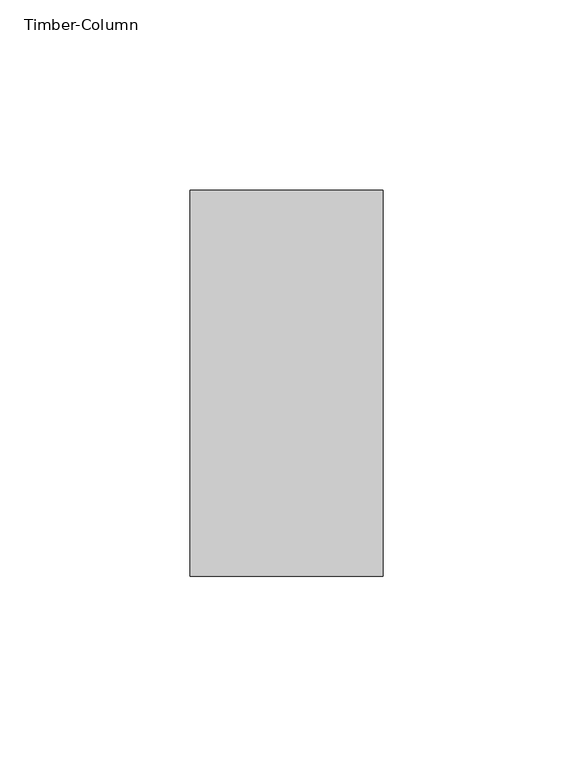
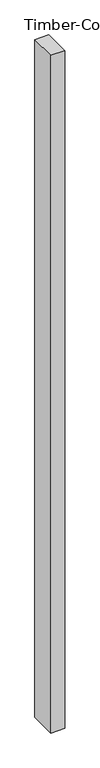
"""IFC4 building model written with IfcOpenShell, lengths in millimetres: column geometry, Timber-Column."""

import ifcopenshell
import ifcopenshell.guid

model = None  # the IFC model being written
_history = None  # IfcOwnerHistory: only IFC2X3 demands one
_inside = {}  # id of a spatial element -> (the spatial element, [elements in it])
_under = {}  # id of a project, library or spatial element -> (it, [spatial elements below it])
_declared = {}  # id of a project -> (the project, [libraries it declares])
_typed = {}  # id of a type object -> (the type object, [elements of that type])
_made_of = {}  # id of a material, layer set ... -> (it, [elements and type objects made of it])


def new_model(schema):
    """Start an empty IFC model of exactly this schema.

    Asked for "IFC4X3", IfcOpenShell would pick the latest addendum, in which some entities
    have other attributes; the version numbers below select the first issue.
    IFC2X3 requires an IfcOwnerHistory on every rooted entity: one is made here for all.
    """
    global model, _history
    if schema == "IFC4X3":
        model = ifcopenshell.file(schema_version=(4, 3, 0, 0))
    else:
        model = ifcopenshell.file(schema=schema)
    _inside.clear()
    _under.clear()
    _declared.clear()
    _typed.clear()
    _made_of.clear()
    _history = None
    if model.schema == "IFC2X3":
        org = make("IfcOrganization", Name="unknown")
        user = make(
            "IfcPersonAndOrganization",
            ThePerson=make("IfcPerson", FamilyName="unknown"),
            TheOrganization=org,
        )
        app = make(
            "IfcApplication",
            ApplicationDeveloper=org,
            Version="unknown",
            ApplicationFullName="unknown",
            ApplicationIdentifier="unknown",
        )
        _history = make(
            "IfcOwnerHistory",
            OwningUser=user,
            OwningApplication=app,
            ChangeAction="ADDED",
            CreationDate=0,
        )
    return model


def make(cls, **values):
    """One entity of the class cls with the attributes given. An attribute that is None is left unset."""
    return model.create_entity(
        cls, **{name: value for name, value in values.items() if value is not None}
    )


def rooted(cls, **values):
    """An entity with a GlobalId (a new one), such as an element, a storey or a relation."""
    return make(cls, GlobalId=ifcopenshell.guid.new(), OwnerHistory=_history, **values)


def si_unit(unit_type, name, prefix=None):
    """IfcSIUnit, for example si_unit("LENGTHUNIT", "METRE", prefix="MILLI")."""
    return make("IfcSIUnit", UnitType=unit_type, Prefix=prefix, Name=name)


def assignment(units):
    """IfcUnitAssignment: the units of a project."""
    return None if units is None else make("IfcUnitAssignment", Units=units)


def point(xyz):
    """IfcCartesianPoint."""
    return None if xyz is None else make("IfcCartesianPoint", Coordinates=xyz)


def direction(xyz):
    """IfcDirection."""
    return None if xyz is None else make("IfcDirection", DirectionRatios=xyz)


def frame(location, z_axis=None, x_axis=None):
    """IfcAxis2Placement3D, a coordinate frame: its origin and axes. An axis left out is left unset."""
    return make(
        "IfcAxis2Placement3D",
        Location=point(location),
        Axis=direction(z_axis),
        RefDirection=direction(x_axis),
    )


def origin():
    """The frame at (0, 0, 0) with its axes left unset."""
    return frame((0.0, 0.0, 0.0))


def place(relative_to, where):
    """IfcLocalPlacement: puts the frame where relative to a parent placement (None: the world)."""
    return make(
        "IfcLocalPlacement", PlacementRelTo=relative_to, RelativePlacement=where
    )


def context(
    kind, dimensions, precision=None, world=None, true_north=None, identifier=None
):
    """IfcGeometricRepresentationContext, for example the 3D "Model" context."""
    return make(
        "IfcGeometricRepresentationContext",
        ContextIdentifier=identifier,
        ContextType=kind,
        CoordinateSpaceDimension=dimensions,
        Precision=precision,
        WorldCoordinateSystem=world,
        TrueNorth=true_north,
    )


def project(units=None, contexts=None):
    """IfcProject with its units and contexts."""
    return rooted(
        "IfcProject",
        Name="project",
        RepresentationContexts=contexts,
        UnitsInContext=assignment(units),
    )


def spatial(cls, under=None, at=None, **own):
    """A site, building, storey or space (cls), placed at a placement, below another one or the project."""
    s = rooted(cls, ObjectPlacement=at, **own)
    if under is not None:
        _under.setdefault(under.id(), (under, []))[1].append(s)
    return s


def polyline(points):
    """IfcPolyline through the points."""
    return make("IfcPolyline", Points=[point(p) for p in points])


def outline(outer, holes=None, kind="AREA"):
    """IfcArbitraryClosedProfileDef: a profile drawn as a closed curve; with holes, ...WithVoids."""
    if holes is None:
        return make("IfcArbitraryClosedProfileDef", ProfileType=kind, OuterCurve=outer)
    return make(
        "IfcArbitraryProfileDefWithVoids",
        ProfileType=kind,
        OuterCurve=outer,
        InnerCurves=holes,
    )


def extrude(swept, where, along, depth):
    """IfcExtrudedAreaSolid: the profile swept, set in the frame where, extruded along a direction by depth."""
    return make(
        "IfcExtrudedAreaSolid",
        SweptArea=swept,
        Position=where,
        ExtrudedDirection=direction(along),
        Depth=depth,
    )


def shape(context_of_items, identifier, shape_type, items):
    """IfcShapeRepresentation: the items that make up one representation, for example the "Body"."""
    return make(
        "IfcShapeRepresentation",
        ContextOfItems=context_of_items,
        RepresentationIdentifier=identifier,
        RepresentationType=shape_type,
        Items=items,
    )


def source(mapping_origin, context_of_items, identifier, shape_type, items):
    """IfcRepresentationMap: a shape defined once, which mapped items show again and again."""
    return make(
        "IfcRepresentationMap",
        MappingOrigin=mapping_origin,
        MappedRepresentation=shape(context_of_items, identifier, shape_type, items),
    )


def transform(
    local_origin,
    x_axis=None,
    y_axis=None,
    z_axis=None,
    scale=None,
    scale2=None,
    scale3=None,
    uniform=True,
):
    """IfcCartesianTransformationOperator3D, or its non-uniform kind. x_axis, y_axis, z_axis: its Axis1, 2, 3."""
    if uniform:
        return make(
            "IfcCartesianTransformationOperator3D",
            Axis1=direction(x_axis),
            Axis2=direction(y_axis),
            LocalOrigin=point(local_origin),
            Scale=scale,
            Axis3=direction(z_axis),
        )
    return make(
        "IfcCartesianTransformationOperator3DnonUniform",
        Axis1=direction(x_axis),
        Axis2=direction(y_axis),
        LocalOrigin=point(local_origin),
        Scale=scale,
        Axis3=direction(z_axis),
        Scale2=scale2,
        Scale3=scale3,
    )


def mapped(mapping_source, mapping_target):
    """IfcMappedItem: shows the shape of a source again, moved by a transform."""
    return make(
        "IfcMappedItem", MappingSource=mapping_source, MappingTarget=mapping_target
    )


def made_of(thing, what):
    """Note that an element or type object is made of a material, layer set ...; save() writes the relation."""
    if what is not None:
        _made_of.setdefault(what.id(), (what, []))[1].append(thing)
    return thing


def element(
    cls,
    number,
    at=None,
    inside=None,
    cuts=None,
    type_object=None,
    material=None,
    context=None,
    identifier="Body",
    shape_type=None,
    held_by="IfcProductDefinitionShape",
    body=None,
    shapes=None,
    **own,
):
    """One element of the class cls, such as IfcWall. Its Tag is "e" and its number.

    at: its placement. inside: the storey or other place that contains it. cuts: it is an
    opening in that element (IfcRelVoidsElement). A single representation is given by context,
    identifier, shape_type and body (its items); several are given by shapes. held_by: the class
    of the entity that holds the representations. save() writes the other relations.
    """
    e = rooted(cls, Tag="e%d" % number, ObjectPlacement=at, **own)
    if body is not None:
        shapes = [shape(context, identifier, shape_type, body)]
    if shapes is not None:
        e.Representation = make(held_by, Representations=shapes)
    if inside is not None:
        _inside.setdefault(inside.id(), (inside, []))[1].append(e)
    if cuts is not None:
        rooted(
            "IfcRelVoidsElement", RelatingBuildingElement=cuts, RelatedOpeningElement=e
        )
    if type_object is not None:
        _typed.setdefault(type_object.id(), (type_object, []))[1].append(e)
    return made_of(e, material)


def aggregate(whole, parts):
    """IfcRelAggregates: a whole, such as a stair, and the parts it consists of."""
    return rooted("IfcRelAggregates", RelatingObject=whole, RelatedObjects=parts)


def save(model, path):
    """Write the relations noted so far, then the file.

    IfcRelAggregates (storeys below a building ...), IfcRelContainedInSpatialStructure (elements
    in a storey), IfcRelDefinesByType, IfcRelAssociatesMaterial and IfcRelDeclares: one each for
    every whole, place, type object, material and project.
    """
    for whole, parts in _under.values():
        aggregate(whole, parts)
    for where, things in _inside.values():
        rooted(
            "IfcRelContainedInSpatialStructure",
            RelatedElements=things,
            RelatingStructure=where,
        )
    for kind, things in _typed.values():
        rooted("IfcRelDefinesByType", RelatedObjects=things, RelatingType=kind)
    for what, things in _made_of.values():
        rooted("IfcRelAssociatesMaterial", RelatedObjects=things, RelatingMaterial=what)
    for by, libraries in _declared.values():
        rooted("IfcRelDeclares", RelatingContext=by, RelatedDefinitions=libraries)
    model.write(path)


def timber_column_c014de30(model_context):
    return source(origin(), model_context, "Body", "SweptSolid", [
        extrude(outline(polyline([(25.4, -50.8), (-25.4, -50.8), (-25.4, 50.8), (25.4, 50.8), (25.4, -50.8)])), frame((0.0, 0.0, 50.8), z_axis=(0.0, 0.0, 1.0), x_axis=(1.0, 0.0, 0.0)), (0.0, 0.0, 1.0), 2616.2),
    ])


if __name__ == "__main__":
    model = new_model("IFC4")
    model_context = context("Model", 3, world=origin())
    ifc_project = project(units=[si_unit("LENGTHUNIT", "METRE", prefix="MILLI")], contexts=[model_context])
    site = spatial("IfcSite", under=ifc_project)
    building = spatial("IfcBuilding", under=site)
    placement = place(None, origin())
    timber_column_shape = timber_column_c014de30(model_context)
    element("IfcColumn", 1, ObjectType="Timber-Column : BLDG 6241 Wall Struds 2\"x4\"", at=placement, inside=building, context=model_context, shape_type="MappedRepresentation", body=[
        mapped(timber_column_shape, transform((0.0, 0.0, 0.0), x_axis=(1.0, 0.0, 0.0), y_axis=(0.0, 1.0, 0.0), z_axis=(0.0, 0.0, 1.0))),
    ])
    save(model, "model.ifc")

# Revit data of these elements
# Type "Timber-Column : BLDG 6241 Wall Struds 2\"x4\""
#   Assembly Code = "B10"
#   A = 0.140625 SF
#   b = 0' - 2"
#   d = 0' - 4"
#   Structural Material [instance default] = Softwood, Lumber
# Element 1 (IfcColumn, "Timber-Column : BLDG 6241 Wall Struds 2\"x4\"")
#   Materials on its faces: "Softwood, Lumber"
# Materials
#   "Softwood, Lumber": class "Wood", colour RGB 223 192 134, transparency 0, Description = "Pinus Echinata", Cost = 0
